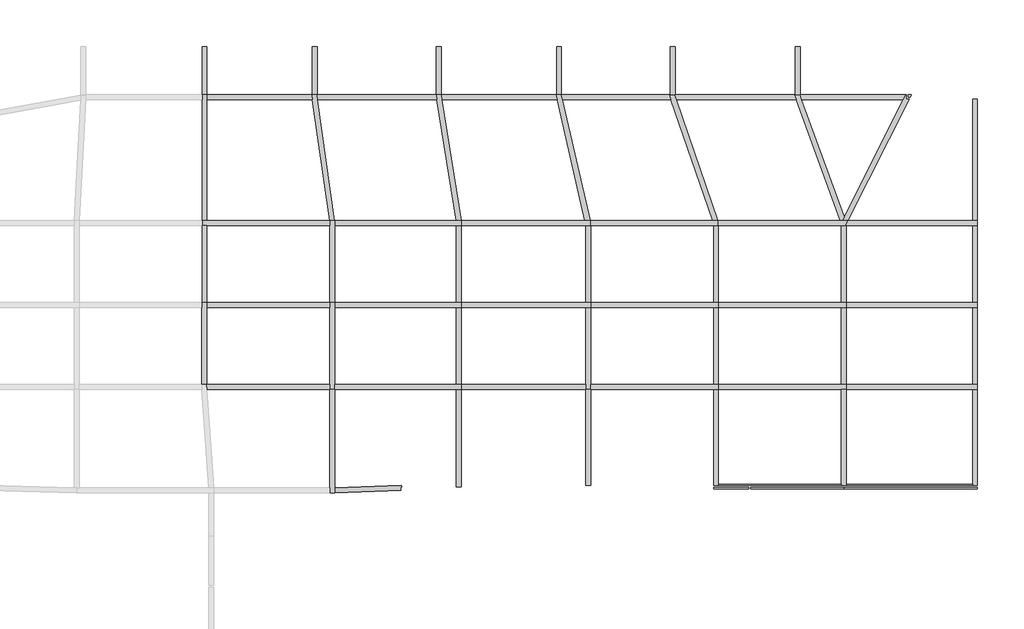
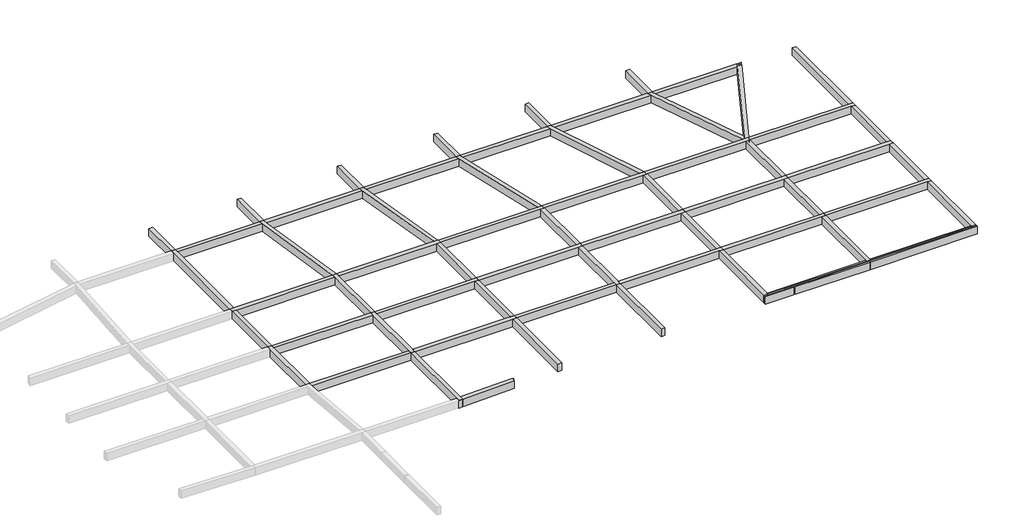
# One storey, part 15 of 15: 61 beams.
"""IFC4 building model written with IfcOpenShell, lengths in millimetres."""

from ifc_helpers import new_model, si_unit, frame, origin, place, context, project, spatial, polyline, outline, extrude, faceted_brep, element, save

model = new_model("IFC4")

# Units and contexts
model_context = context("Model", 3, world=origin())
ifc_project = project(units=[si_unit("LENGTHUNIT", "METRE", prefix="MILLI")], contexts=[model_context])

# Site, building, storey
site = spatial("IfcSite", under=ifc_project)
building = spatial("IfcBuilding", under=site)
storey = spatial("IfcBuildingStorey", under=building, Name="层高", Elevation=3300.0)

# Beams
placement = place(None, origin())
element("IfcBeam", 1, ObjectType="混凝土 - 矩形梁 : KL_beam", at=placement, inside=storey, context=model_context, shape_type="Brep", body=[
    faceted_brep([(266349.8041274, 106691.6486698, 3300.0), (266649.8041274, 106691.6486698, 3300.0), (266649.8041274, 106991.6486698, 3300.0), (266649.8041274, 111691.6486698, 3300.0), (266649.8041274, 111991.6486698, 3300.0), (266349.8041274, 111991.6486698, 3300.0), (266349.8041274, 111691.6486698, 3300.0), (266349.8041274, 106991.6486698, 3300.0), (266649.8041274, 106691.6486698, 2700.0), (266649.8041274, 106991.6486698, 2700.0), (266649.8041274, 111691.6486698, 2700.0), (266649.8041274, 111991.6486698, 2700.0), (266349.8041274, 106691.6486698, 2700.0), (266349.8041274, 106991.6486698, 2700.0), (266349.8041274, 111691.6486698, 2700.0), (266349.8041274, 111991.6486698, 2700.0)], [[[0, 1, 2, 3, 4, 5, 6, 7]], [[1, 8, 9, 10, 11, 4, 3, 2]], [[8, 12, 13, 14, 15, 11, 10, 9]], [[12, 0, 7, 6, 5, 15, 14, 13]], [[1, 0, 12, 8]], [[5, 4, 11, 15]]]),
])
element("IfcBeam", 2, ObjectType="混凝土 - 矩形梁 : KL_beam", at=placement, inside=storey, context=model_context, shape_type="Brep", body=[
    faceted_brep([(274370.4678588, 106691.6486698, 3300.0), (274370.4678588, 106991.6486698, 3300.0), (274070.4678588, 106991.6486698, 3300.0), (266649.8041274, 106991.6486698, 3300.0), (266649.8041274, 106691.6486698, 3300.0), (274070.4678588, 106691.6486698, 3300.0), (274370.4678588, 106991.6486698, 2700.0), (274070.4678588, 106991.6486698, 2700.0), (266649.8041274, 106991.6486698, 2700.0), (274370.4678588, 106691.6486698, 2700.0), (274070.4678588, 106691.6486698, 2700.0), (266649.8041274, 106691.6486698, 2700.0)], [[[0, 1, 2, 3, 4, 5]], [[1, 6, 7, 8, 3, 2]], [[6, 9, 10, 11, 8, 7]], [[9, 0, 5, 4, 11, 10]], [[4, 3, 8, 11]], [[1, 0, 9, 6]]]),
])
element("IfcBeam", 3, ObjectType="混凝土 - 矩形梁 : KL_beam", at=placement, inside=storey, context=model_context, shape_type="Brep", body=[
    faceted_brep([(274370.4678588, 111691.6486698, 3300.0), (274370.4678588, 111991.6486698, 3300.0), (274070.4678588, 111991.6486698, 3300.0), (266649.8041274, 111991.6486698, 3300.0), (266649.8041274, 111691.6486698, 3300.0), (274070.4678588, 111691.6486698, 3300.0), (274370.4678588, 111691.6486698, 2700.0), (266649.8041274, 111691.6486698, 2700.0), (274070.4678588, 111691.6486698, 2700.0), (274370.4678588, 111991.6486698, 2700.0), (266649.8041274, 111991.6486698, 2700.0), (274070.4678588, 111991.6486698, 2700.0)], [[[0, 1, 2, 3, 4, 5]], [[6, 0, 5, 4, 7, 8]], [[9, 6, 8, 7, 10, 11]], [[1, 9, 11, 10, 3, 2]], [[4, 3, 10, 7]], [[1, 0, 6, 9]]]),
])
element("IfcBeam", 4, ObjectType="混凝土 - 矩形梁 : KL_beam", at=placement, inside=storey, context=model_context, shape_type="SweptSolid", body=[
    extrude(outline(polyline([(274370.4678588, 106991.6486698), (274070.4678588, 106991.6486698), (274070.4678588, 111691.6486698), (274370.4678588, 111691.6486698), (274370.4678588, 106991.6486698)])), frame((0.0, 0.0, 2700.0), z_axis=(0.0, 0.0, 1.0), x_axis=(1.0, 0.0, 0.0)), (0.0, 0.0, 1.0), 600.0),
])
element("IfcBeam", 5, ObjectType="混凝土 - 矩形梁 : KL_beam", at=placement, inside=storey, context=model_context, shape_type="Brep", body=[
    faceted_brep([(266349.8041274, 100396.7953536, 3300.0), (266649.8041274, 100396.7953536, 3300.0), (266649.8041274, 100696.9782169, 3300.0), (266649.8041274, 106691.6486698, 3300.0), (266349.8041274, 106691.6486698, 3300.0), (266349.8041274, 100691.6486698, 3300.0), (266349.8041274, 100396.7953536, 2700.0), (266349.8041274, 106691.6486698, 2700.0), (266349.8041274, 100691.6486698, 2700.0), (266649.8041274, 100396.7953536, 2700.0), (266649.8041274, 106691.6486698, 2700.0), (266649.8041274, 100696.9782169, 2700.0)], [[[0, 1, 2, 3, 4, 5]], [[6, 0, 5, 4, 7, 8]], [[9, 6, 8, 7, 10, 11]], [[1, 9, 11, 10, 3, 2]], [[4, 3, 10, 7]], [[1, 0, 6, 9]]]),
])
element("IfcBeam", 6, ObjectType="混凝土 - 矩形梁 : KL_beam", at=placement, inside=storey, context=model_context, shape_type="Brep", body=[
    faceted_brep([(270716.2250579, 100838.9807649, 2700.0), (270716.2250579, 100838.9807649, 3300.0), (270719.5879307, 100742.6806889, 3300.0), (270719.5879307, 100742.6806889, 2700.0), (266649.8041274, 100696.9782169, 3300.0), (266649.8041274, 100396.7953536, 3300.0), (270661.6831769, 100536.8932571, 3300.0), (270661.6831769, 100742.6806889, 3300.0), (266349.8041274, 100386.3191227, 3300.0), (266349.8041274, 100386.3191227, 2700.0), (266649.8041274, 100396.7953536, 2700.0), (270661.6831769, 100536.8932571, 2700.0), (266649.8041274, 100696.9782169, 2700.0), (270661.6831769, 100742.6806889, 2700.0), (266349.8041274, 100391.6486698, 3300.0), (266349.8041274, 100396.7953536, 3300.0), (266349.8041274, 100396.7953536, 2700.0), (266349.8041274, 100391.6486698, 2700.0)], [[[0, 1, 2, 3]], [[1, 4, 5, 6, 7, 2]], [[8, 9, 10, 11, 6, 5]], [[12, 0, 3, 13, 11, 10]], [[1, 0, 12, 4]], [[9, 8, 14, 15, 16, 17]], [[10, 5, 4, 12]], [[5, 10, 16, 15]], [[15, 14, 8, 5]], [[10, 9, 17, 16]], [[13, 7, 6, 11]], [[7, 13, 3, 2]]]),
])
element("IfcBeam", 7, ObjectType="混凝土 - 矩形梁 : KL_beam", at=placement, inside=storey, context=model_context, shape_type="SweptSolid", body=[
    extrude(outline(polyline([(274070.4678588, 106691.6486698), (274370.4678588, 106691.6486698), (274370.4678588, 100742.6806889), (274070.4678588, 100742.6806889), (274070.4678588, 106691.6486698)])), frame((0.0, 0.0, 2700.0), z_axis=(0.0, 0.0, 1.0), x_axis=(1.0, 0.0, 0.0)), (0.0, 0.0, 1.0), 600.0),
])
element("IfcBeam", 8, ObjectType="混凝土 - 矩形梁 : KL_beam", at=placement, inside=storey, context=model_context, shape_type="Brep", body=[
    faceted_brep([(266349.8041274, 106691.6486698, 3300.0), (266349.8041274, 106991.6486698, 3300.0), (258831.1501343, 106991.6486698, 3300.0), (258821.0273972, 106991.6486698, 3300.0), (258842.0054408, 106691.6486698, 3300.0), (266349.8041274, 106991.6486698, 2700.0), (258831.1501343, 106991.6486698, 2700.0), (258821.0273972, 106991.6486698, 2700.0), (266349.8041274, 106691.6486698, 2700.0), (258842.0054408, 106691.6486698, 2700.0)], [[[0, 1, 2, 3, 4]], [[1, 5, 6, 7, 3, 2]], [[5, 8, 9, 7, 6]], [[8, 0, 4, 9]], [[1, 0, 8, 5]], [[4, 3, 7, 9]]]),
])
element("IfcBeam", 9, ObjectType="混凝土 - 矩形梁 : KL_beam", at=placement, inside=storey, context=model_context, shape_type="Brep", body=[
    faceted_brep([(258831.1501343, 106991.6486698, 3300.0), (258831.1501343, 106991.6486698, 2700.0), (258831.1501343, 111691.6486698, 2700.0), (258831.1501343, 111991.6486698, 2700.0), (258831.1501343, 111991.6486698, 3300.0), (258831.1501343, 111691.6486698, 3300.0), (258549.8041274, 111991.6486698, 3300.0), (258531.1501343, 111991.6486698, 3300.0), (258531.1501343, 111691.6486698, 3300.0), (258531.1501343, 106991.6486698, 3300.0), (258821.0273972, 106991.6486698, 3300.0), (258531.1501343, 111991.6486698, 2700.0), (258549.8041274, 111991.6486698, 2700.0), (258821.0273972, 106991.6486698, 2700.0), (258531.1501343, 106991.6486698, 2700.0), (258531.1501343, 111691.6486698, 2700.0)], [[[0, 1, 2, 3, 4, 5]], [[4, 6, 7, 8, 9, 10, 0, 5]], [[11, 12, 3, 2, 1, 13, 14, 15]], [[7, 11, 15, 14, 9, 8]], [[1, 0, 10, 9, 14, 13]], [[7, 6, 4, 3, 12, 11]]]),
])
element("IfcBeam", 10, ObjectType="混凝土 - 矩形梁 : KL_beam", at=placement, inside=storey, context=model_context, shape_type="Brep", body=[
    faceted_brep([(266349.8041274, 111691.6486698, 3300.0), (266349.8041274, 111991.6486698, 3300.0), (258849.8041274, 111991.6486698, 3300.0), (258831.1501343, 111991.6486698, 3300.0), (258831.1501343, 111691.6486698, 3300.0), (266349.8041274, 111691.6486698, 2700.0), (258831.1501343, 111691.6486698, 2700.0), (266349.8041274, 111991.6486698, 2700.0), (258831.1501343, 111991.6486698, 2700.0), (258849.8041274, 111991.6486698, 2700.0)], [[[0, 1, 2, 3, 4]], [[5, 0, 4, 6]], [[7, 5, 6, 8, 9]], [[1, 7, 9, 8, 3, 2]], [[1, 0, 5, 7]], [[4, 3, 8, 6]]]),
])
element("IfcBeam", 11, ObjectType="混凝土 - 矩形梁 : KL_beam", at=placement, inside=storey, context=model_context, shape_type="Brep", body=[
    faceted_brep([(266649.8041274, 116991.6486698, 3300.0), (266630.197138, 116991.6486698, 3300.0), (266349.8041274, 116991.6486698, 3300.0), (266349.8041274, 116691.6486698, 3300.0), (266349.8041274, 111991.6486698, 3300.0), (266649.8041274, 111991.6486698, 3300.0), (266649.8041274, 116691.6486698, 3300.0), (266649.8041274, 116852.1376916, 3300.0), (266649.8041274, 116991.6486698, 2700.0), (266649.8041274, 111991.6486698, 2700.0), (266649.8041274, 116691.6486698, 2700.0), (266649.8041274, 116852.1376916, 2700.0), (266349.8041274, 116991.6486698, 2700.0), (266630.197138, 116991.6486698, 2700.0), (266349.8041274, 111991.6486698, 2700.0), (266349.8041274, 116691.6486698, 2700.0)], [[[0, 1, 2, 3, 4, 5, 6, 7]], [[8, 0, 7, 6, 5, 9, 10, 11]], [[12, 13, 8, 11, 10, 9, 14, 15]], [[2, 12, 15, 14, 4, 3]], [[5, 4, 14, 9]], [[2, 1, 0, 8, 13, 12]]]),
])
element("IfcBeam", 12, ObjectType="混凝土 - 矩形梁 : KL_beam", at=placement, inside=storey, context=model_context, shape_type="Brep", body=[
    faceted_brep([(258549.8041274, 116991.6486698, 3300.0), (258549.8041274, 116691.6486698, 3300.0), (258849.8041274, 116691.6486698, 3300.0), (266349.8041274, 116691.6486698, 3300.0), (266349.8041274, 116991.6486698, 3300.0), (266327.2488663, 116991.6486698, 3300.0), (258849.8041274, 116991.6486698, 3300.0), (258549.8041274, 116991.6486698, 2700.0), (266349.8041274, 116991.6486698, 2700.0), (266327.2488663, 116991.6486698, 2700.0), (258849.8041274, 116991.6486698, 2700.0), (258549.8041274, 116691.6486698, 2700.0), (266349.8041274, 116691.6486698, 2700.0), (258849.8041274, 116691.6486698, 2700.0)], [[[0, 1, 2, 3, 4, 5, 6]], [[7, 0, 6, 5, 4, 8, 9, 10]], [[11, 7, 10, 9, 8, 12, 13]], [[1, 11, 13, 12, 3, 2]], [[4, 3, 12, 8]], [[1, 0, 7, 11]]]),
])
element("IfcBeam", 13, ObjectType="混凝土 - 矩形梁 : KL_beam", at=placement, inside=storey, context=model_context, shape_type="Brep", body=[
    faceted_brep([(258549.8041274, 111991.6486698, 3300.0), (258831.1501343, 111991.6486698, 3300.0), (258849.8041274, 111991.6486698, 3300.0), (258849.8041274, 116691.6486698, 3300.0), (258549.8041274, 116691.6486698, 3300.0), (258549.8041274, 111991.6486698, 2700.0), (258549.8041274, 116691.6486698, 2700.0), (258849.8041274, 111991.6486698, 2700.0), (258831.1501343, 111991.6486698, 2700.0), (258849.8041274, 116691.6486698, 2700.0)], [[[0, 1, 2, 3, 4]], [[5, 0, 4, 6]], [[7, 8, 5, 6, 9]], [[2, 7, 9, 3]], [[0, 5, 8, 7, 2, 1]], [[4, 3, 9, 6]]]),
])
element("IfcBeam", 14, ObjectType="混凝土 - 矩形梁 : KL_beam", at=placement, inside=storey, context=model_context, shape_type="Brep", body=[
    faceted_brep([(258849.8041274, 124681.0960874, 3300.0), (258549.8041274, 124681.0960874, 3300.0), (258549.8041274, 124381.0960874, 3300.0), (258549.8041274, 116991.6486698, 3300.0), (258849.8041274, 116991.6486698, 3300.0), (258849.8041274, 124381.0960874, 3300.0), (258849.8041274, 124681.0960874, 2700.0), (258849.8041274, 116991.6486698, 2700.0), (258849.8041274, 124381.0960874, 2700.0), (258549.8041274, 124681.0960874, 2700.0), (258549.8041274, 116991.6486698, 2700.0), (258549.8041274, 124381.0960874, 2700.0)], [[[0, 1, 2, 3, 4, 5]], [[6, 0, 5, 4, 7, 8]], [[9, 6, 8, 7, 10, 11]], [[1, 9, 11, 10, 3, 2]], [[4, 3, 10, 7]], [[1, 0, 6, 9]]]),
])
element("IfcBeam", 15, ObjectType="混凝土 - 矩形梁 : KL_beam", at=placement, inside=storey, context=model_context, shape_type="Brep", body=[
    faceted_brep([(266327.2488663, 116991.6486698, 3300.0), (266349.8041274, 116991.6486698, 3300.0), (266630.197138, 116991.6486698, 3300.0), (265591.67803, 124381.0960874, 3300.0), (265549.5157796, 124681.0960874, 3300.0), (265269.1227689, 124681.0960874, 3300.0), (265246.5675078, 124681.0960874, 3300.0), (265288.7297582, 124381.0960874, 3300.0), (266630.197138, 116991.6486698, 2700.0), (265591.67803, 124381.0960874, 2700.0), (265549.5157796, 124681.0960874, 2700.0), (266349.8041274, 116991.6486698, 2700.0), (266327.2488663, 116991.6486698, 2700.0), (265288.7297582, 124381.0960874, 2700.0), (265246.5675078, 124681.0960874, 2700.0), (265269.1227689, 124681.0960874, 2700.0)], [[[0, 1, 2, 3, 4, 5, 6, 7]], [[2, 8, 9, 10, 4, 3]], [[8, 11, 12, 13, 14, 15, 10, 9]], [[6, 14, 13, 12, 0, 7]], [[0, 12, 11, 8, 2, 1]], [[6, 5, 4, 10, 15, 14]]]),
    faceted_brep([(266672.3593884, 116691.6486698, 2700.0), (266672.3593884, 116691.6486698, 3300.0), (266649.8041274, 116691.6486698, 3300.0), (266649.8041274, 116691.6486698, 2700.0), (266649.8041274, 116852.1376916, 3300.0), (266649.8041274, 116852.1376916, 2700.0)], [[[0, 1, 2, 3]], [[2, 4, 5, 3]], [[4, 2, 1]], [[1, 0, 5, 4]], [[3, 5, 0]]]),
])
element("IfcBeam", 16, ObjectType="混凝土 - 矩形梁 : KL_beam", at=placement, inside=storey, context=model_context, shape_type="Brep", body=[
    faceted_brep([(274370.4678588, 116691.6486698, 3300.0), (274370.4678588, 116991.6486698, 3300.0), (274348.5799616, 116991.6486698, 3300.0), (274044.8404239, 116991.6486698, 3300.0), (266649.8041274, 116991.6486698, 3300.0), (266649.8041274, 116852.1376916, 3300.0), (266672.3593884, 116691.6486698, 3300.0), (274070.4678588, 116691.6486698, 3300.0), (274370.4678588, 116691.6486698, 2700.0), (266672.3593884, 116691.6486698, 2700.0), (274070.4678588, 116691.6486698, 2700.0), (274370.4678588, 116991.6486698, 2700.0), (266649.8041274, 116852.1376916, 2700.0), (266649.8041274, 116991.6486698, 2700.0), (274044.8404239, 116991.6486698, 2700.0), (274348.5799616, 116991.6486698, 2700.0)], [[[0, 1, 2, 3, 4, 5, 6, 7]], [[8, 0, 7, 6, 9, 10]], [[11, 8, 10, 9, 12, 13, 14, 15]], [[13, 4, 3, 2, 1, 11, 15, 14]], [[4, 13, 12, 5]], [[6, 5, 12, 9]], [[1, 0, 8, 11]]]),
])
element("IfcBeam", 17, ObjectType="混凝土 - 矩形梁 : KL_beam", at=placement, inside=storey, context=model_context, shape_type="SweptSolid", body=[
    extrude(outline(polyline([(274370.4678588, 111991.6486698), (274070.4678588, 111991.6486698), (274070.4678588, 116691.6486698), (274370.4678588, 116691.6486698), (274370.4678588, 111991.6486698)])), frame((0.0, 0.0, 2700.0), z_axis=(0.0, 0.0, 1.0), x_axis=(1.0, 0.0, 0.0)), (0.0, 0.0, 1.0), 600.0),
])
element("IfcBeam", 18, ObjectType="混凝土 - 矩形梁 : KL_beam", at=placement, inside=storey, context=model_context, shape_type="Brep", body=[
    faceted_brep([(282219.0254303, 116691.6486698, 3300.0), (282219.0254303, 116991.6486698, 3300.0), (281911.134198, 116991.6486698, 3300.0), (274370.4678588, 116991.6486698, 3300.0), (274370.4678588, 116691.6486698, 3300.0), (281949.7100428, 116691.6486698, 3300.0), (282219.0254303, 116691.6486698, 2700.0), (274370.4678588, 116691.6486698, 2700.0), (281949.7100428, 116691.6486698, 2700.0), (282219.0254303, 116991.6486698, 2700.0), (274370.4678588, 116991.6486698, 2700.0), (281911.134198, 116991.6486698, 2700.0)], [[[0, 1, 2, 3, 4, 5]], [[6, 0, 5, 4, 7, 8]], [[9, 6, 8, 7, 10, 11]], [[1, 9, 11, 10, 3, 2]], [[4, 3, 10, 7]], [[1, 0, 6, 9]]]),
])
element("IfcBeam", 19, ObjectType="混凝土 - 矩形梁 : KL_beam", at=placement, inside=storey, context=model_context, shape_type="Brep", body=[
    faceted_brep([(290006.8166962, 116691.6486698, 3300.0), (290006.8166962, 116991.6486698, 3300.0), (289689.5304919, 116991.6486698, 3300.0), (282219.0254303, 116991.6486698, 3300.0), (282219.0254303, 116691.6486698, 3300.0), (282249.7100428, 116691.6486698, 3300.0), (289749.8227361, 116691.6486698, 3300.0), (290006.8166962, 116691.6486698, 2700.0), (282219.0254303, 116691.6486698, 2700.0), (282249.7100428, 116691.6486698, 2700.0), (289749.8227361, 116691.6486698, 2700.0), (290006.8166962, 116991.6486698, 2700.0), (282219.0254303, 116991.6486698, 2700.0), (289689.5304919, 116991.6486698, 2700.0)], [[[0, 1, 2, 3, 4, 5, 6]], [[7, 0, 6, 5, 4, 8, 9, 10]], [[11, 7, 10, 9, 8, 12, 13]], [[1, 11, 13, 12, 3, 2]], [[4, 3, 12, 8]], [[1, 0, 7, 11]]]),
])
element("IfcBeam", 20, ObjectType="混凝土 - 矩形梁 : KL_beam", at=placement, inside=storey, context=model_context, shape_type="Brep", body=[
    faceted_brep([(297792.1399936, 116691.6486698, 3300.0), (297943.4797534, 116991.6486698, 3300.0), (297607.4682611, 116991.6486698, 3300.0), (297485.5819263, 116991.6486698, 3300.0), (290006.8166962, 116991.6486698, 3300.0), (290006.8166962, 116691.6486698, 3300.0), (290049.8227361, 116691.6486698, 3300.0), (297549.8041274, 116691.6486698, 3300.0), (297792.1399936, 116691.6486698, 2700.0), (290006.8166962, 116691.6486698, 2700.0), (290049.8227361, 116691.6486698, 2700.0), (297549.8041274, 116691.6486698, 2700.0), (297943.4797534, 116991.6486698, 2700.0), (290006.8166962, 116991.6486698, 2700.0), (297485.5819263, 116991.6486698, 2700.0), (297607.4682611, 116991.6486698, 2700.0)], [[[0, 1, 2, 3, 4, 5, 6, 7]], [[8, 0, 7, 6, 5, 9, 10, 11]], [[12, 8, 11, 10, 9, 13, 14, 15]], [[1, 12, 15, 14, 13, 4, 3, 2]], [[5, 4, 13, 9]], [[1, 0, 8, 12]]]),
])
element("IfcBeam", 21, ObjectType="混凝土 - 矩形梁 : KL_beam", at=placement, inside=storey, context=model_context, shape_type="Brep", body=[
    faceted_brep([(297943.4797534, 116991.6486698, 3300.0), (297792.1399936, 116691.6486698, 3300.0), (297849.8041274, 116691.6486698, 3300.0), (305549.8041274, 116691.6486698, 3300.0), (305849.8041274, 116691.6486698, 3300.0), (305849.8041274, 116991.6486698, 3300.0), (305549.8041274, 116991.6486698, 3300.0), (297792.1399936, 116691.6486698, 2700.0), (297849.8041274, 116691.6486698, 2700.0), (305549.8041274, 116691.6486698, 2700.0), (305849.8041274, 116691.6486698, 2700.0), (297943.4797534, 116991.6486698, 2700.0), (305549.8041274, 116991.6486698, 2700.0), (305849.8041274, 116991.6486698, 2700.0)], [[[0, 1, 2, 3, 4, 5, 6]], [[1, 7, 8, 9, 10, 4, 3, 2]], [[7, 11, 12, 13, 10, 9, 8]], [[11, 0, 6, 5, 13, 12]], [[1, 0, 11, 7]], [[5, 4, 10, 13]]]),
])
element("IfcBeam", 22, ObjectType="混凝土 - 矩形梁 : KL_beam", at=placement, inside=storey, context=model_context, shape_type="Brep", body=[
    faceted_brep([(301822.5435038, 124681.0960874, 3300.0), (301617.9590704, 124681.0960874, 3300.0), (301617.9590704, 124549.6486698, 3300.0), (301756.2327685, 124549.6486698, 3300.0), (301822.5435038, 124681.0960874, 2700.0), (301756.2327685, 124549.6486698, 2700.0), (301617.9590704, 124681.0960874, 2700.0), (301617.9590704, 124549.6486698, 2700.0)], [[[0, 1, 2, 3]], [[4, 0, 3, 5]], [[6, 4, 5, 7]], [[1, 6, 7, 2]], [[3, 2, 7, 5]], [[0, 4, 6, 1]]]),
    faceted_brep([(297607.4682611, 116991.6486698, 2700.0), (297607.4682611, 116991.6486698, 3300.0), (297722.1167805, 117218.9158192, 3300.0), (301335.1922518, 124381.0960874, 3300.0), (301486.5320116, 124681.0960874, 3300.0), (301486.5320116, 124681.0960874, 2700.0), (301335.1922518, 124381.0960874, 2700.0), (297722.1167805, 117218.9158192, 2700.0), (297943.4797534, 116991.6486698, 3300.0), (297943.4797534, 116991.6486698, 2700.0), (301497.9590704, 124681.0960874, 3300.0), (301497.9590704, 124681.0960874, 2700.0), (301497.9590704, 124429.6486698, 3300.0), (301497.9590704, 124429.6486698, 2700.0), (301695.6968645, 124429.6486698, 3300.0), (301695.6968645, 124429.6486698, 2700.0)], [[[0, 1, 2, 3, 4, 5, 6, 7]], [[8, 1, 0, 9]], [[5, 4, 10, 11]], [[12, 13, 11, 10]], [[13, 12, 14, 15]], [[1, 8, 14, 12, 10, 4, 3, 2]], [[8, 9, 15, 14]], [[9, 0, 7, 6, 5, 11, 13, 15]]]),
])
element("IfcBeam", 23, ObjectType="混凝土 - 矩形梁 : KL_beam", at=placement, inside=storey, context=model_context, shape_type="Brep", body=[
    faceted_brep([(297485.5819263, 116991.6486698, 3300.0), (297607.4682611, 116991.6486698, 3300.0), (297722.1167805, 117218.9158192, 3300.0), (295115.2963504, 124381.0960874, 3300.0), (295006.1052801, 124681.0960874, 3300.0), (294751.0741494, 124681.0960874, 3300.0), (294686.8519484, 124681.0960874, 3300.0), (294796.0430187, 124381.0960874, 3300.0), (297722.1167805, 117218.9158192, 2700.0), (295115.2963504, 124381.0960874, 2700.0), (295006.1052801, 124681.0960874, 2700.0), (297607.4682611, 116991.6486698, 2700.0), (297485.5819263, 116991.6486698, 2700.0), (294796.0430187, 124381.0960874, 2700.0), (294686.8519484, 124681.0960874, 2700.0), (294751.0741494, 124681.0960874, 2700.0)], [[[0, 1, 2, 3, 4, 5, 6, 7]], [[2, 8, 9, 10, 4, 3]], [[11, 12, 13, 14, 15, 10, 9, 8]], [[12, 0, 7, 6, 14, 13]], [[0, 12, 11, 1]], [[2, 1, 11, 8]], [[6, 5, 4, 10, 15, 14]]]),
])
element("IfcBeam", 24, ObjectType="混凝土 - 矩形梁 : KL_beam", at=placement, inside=storey, context=model_context, shape_type="Brep", body=[
    faceted_brep([(287359.1276194, 124681.0960874, 3300.0), (287102.1336592, 124681.0960874, 3300.0), (287041.8414151, 124681.0960874, 3300.0), (287145.139699, 124381.0960874, 3300.0), (289689.5304919, 116991.6486698, 3300.0), (290006.8166962, 116991.6486698, 3300.0), (287462.4259034, 124381.0960874, 3300.0), (287359.1276194, 124681.0960874, 2700.0), (290006.8166962, 116991.6486698, 2700.0), (287462.4259034, 124381.0960874, 2700.0), (287041.8414151, 124681.0960874, 2700.0), (287102.1336592, 124681.0960874, 2700.0), (289689.5304919, 116991.6486698, 2700.0), (287145.139699, 124381.0960874, 2700.0)], [[[0, 1, 2, 3, 4, 5, 6]], [[7, 0, 6, 5, 8, 9]], [[10, 11, 7, 9, 8, 12, 13]], [[2, 10, 13, 12, 4, 3]], [[5, 4, 12, 8]], [[2, 1, 0, 7, 11, 10]]]),
])
element("IfcBeam", 25, ObjectType="混凝土 - 矩形梁 : KL_beam", at=placement, inside=storey, context=model_context, shape_type="Brep", body=[
    faceted_brep([(280443.7766143, 124681.0960874, 3300.0), (280174.4612268, 124681.0960874, 3300.0), (280135.8853819, 124681.0960874, 3300.0), (280205.1458393, 124381.0960874, 3300.0), (281911.134198, 116991.6486698, 3300.0), (282219.0254303, 116991.6486698, 3300.0), (280513.0370716, 124381.0960874, 3300.0), (280443.7766143, 124681.0960874, 2700.0), (282219.0254303, 116991.6486698, 2700.0), (280513.0370716, 124381.0960874, 2700.0), (280135.8853819, 124681.0960874, 2700.0), (280174.4612268, 124681.0960874, 2700.0), (281911.134198, 116991.6486698, 2700.0), (280205.1458393, 124381.0960874, 2700.0)], [[[0, 1, 2, 3, 4, 5, 6]], [[7, 0, 6, 5, 8, 9]], [[10, 11, 7, 9, 8, 12, 13]], [[2, 10, 13, 12, 4, 3]], [[5, 4, 12, 8]], [[2, 1, 0, 7, 11, 10]]]),
])
element("IfcBeam", 26, ObjectType="混凝土 - 矩形梁 : KL_beam", at=placement, inside=storey, context=model_context, shape_type="Brep", body=[
    faceted_brep([(274044.8404239, 116991.6486698, 3300.0), (274070.4678588, 116991.6486698, 3300.0), (274348.5799616, 116991.6486698, 3300.0), (273178.2064681, 124381.0960874, 3300.0), (273130.691136, 124681.0960874, 3300.0), (272852.5790331, 124681.0960874, 3300.0), (272826.9515982, 124681.0960874, 3300.0), (272874.4669303, 124381.0960874, 3300.0), (274348.5799616, 116991.6486698, 2700.0), (273178.2064681, 124381.0960874, 2700.0), (273130.691136, 124681.0960874, 2700.0), (274070.4678588, 116991.6486698, 2700.0), (274044.8404239, 116991.6486698, 2700.0), (272874.4669303, 124381.0960874, 2700.0), (272826.9515982, 124681.0960874, 2700.0), (272852.5790331, 124681.0960874, 2700.0)], [[[0, 1, 2, 3, 4, 5, 6, 7]], [[2, 8, 9, 10, 4, 3]], [[8, 11, 12, 13, 14, 15, 10, 9]], [[12, 0, 7, 6, 14, 13]], [[8, 2, 1, 0, 12, 11]], [[6, 5, 4, 10, 15, 14]]]),
])
element("IfcBeam", 27, ObjectType="混凝土 - 矩形梁 : KL_beam", at=placement, inside=storey, context=model_context, shape_type="Brep", body=[
    faceted_brep([(282249.7100428, 111691.6486698, 3300.0), (282249.7100428, 111991.6486698, 3300.0), (281949.7100428, 111991.6486698, 3300.0), (274370.4678588, 111991.6486698, 3300.0), (274370.4678588, 111691.6486698, 3300.0), (281949.7100428, 111691.6486698, 3300.0), (282249.7100428, 111691.6486698, 2700.0), (274370.4678588, 111691.6486698, 2700.0), (281949.7100428, 111691.6486698, 2700.0), (282249.7100428, 111991.6486698, 2700.0), (274370.4678588, 111991.6486698, 2700.0), (281949.7100428, 111991.6486698, 2700.0)], [[[0, 1, 2, 3, 4, 5]], [[6, 0, 5, 4, 7, 8]], [[9, 6, 8, 7, 10, 11]], [[1, 9, 11, 10, 3, 2]], [[4, 3, 10, 7]], [[1, 0, 6, 9]]]),
])
element("IfcBeam", 28, ObjectType="混凝土 - 矩形梁 : KL_beam", at=placement, inside=storey, context=model_context, shape_type="Brep", body=[
    faceted_brep([(290049.8227361, 111691.6486698, 3300.0), (290049.8227361, 111991.6486698, 3300.0), (289749.8227361, 111991.6486698, 3300.0), (282249.7100428, 111991.6486698, 3300.0), (282249.7100428, 111691.6486698, 3300.0), (289749.8227361, 111691.6486698, 3300.0), (290049.8227361, 111691.6486698, 2700.0), (282249.7100428, 111691.6486698, 2700.0), (289749.8227361, 111691.6486698, 2700.0), (290049.8227361, 111991.6486698, 2700.0), (282249.7100428, 111991.6486698, 2700.0), (289749.8227361, 111991.6486698, 2700.0)], [[[0, 1, 2, 3, 4, 5]], [[6, 0, 5, 4, 7, 8]], [[9, 6, 8, 7, 10, 11]], [[1, 9, 11, 10, 3, 2]], [[1, 0, 6, 9]], [[4, 3, 10, 7]]]),
])
element("IfcBeam", 29, ObjectType="混凝土 - 矩形梁 : KL_beam", at=placement, inside=storey, context=model_context, shape_type="Brep", body=[
    faceted_brep([(297849.8041274, 111691.6486698, 3300.0), (297849.8041274, 111991.6486698, 3300.0), (297549.8041274, 111991.6486698, 3300.0), (290049.8227361, 111991.6486698, 3300.0), (290049.8227361, 111691.6486698, 3300.0), (297549.8041274, 111691.6486698, 3300.0), (297849.8041274, 111691.6486698, 2700.0), (290049.8227361, 111691.6486698, 2700.0), (297549.8041274, 111691.6486698, 2700.0), (297849.8041274, 111991.6486698, 2700.0), (290049.8227361, 111991.6486698, 2700.0), (297549.8041274, 111991.6486698, 2700.0)], [[[0, 1, 2, 3, 4, 5]], [[6, 0, 5, 4, 7, 8]], [[9, 6, 8, 7, 10, 11]], [[1, 9, 11, 10, 3, 2]], [[4, 3, 10, 7]], [[1, 0, 6, 9]]]),
])
element("IfcBeam", 30, ObjectType="混凝土 - 矩形梁 : KL_beam", at=placement, inside=storey, context=model_context, shape_type="Brep", body=[
    faceted_brep([(290049.8227361, 116691.6486698, 3300.0), (290006.8166962, 116691.6486698, 3300.0), (289749.8227361, 116691.6486698, 3300.0), (289749.8227361, 111991.6486698, 3300.0), (290049.8227361, 111991.6486698, 3300.0), (290049.8227361, 116691.6486698, 2700.0), (290049.8227361, 111991.6486698, 2700.0), (289749.8227361, 116691.6486698, 2700.0), (290006.8166962, 116691.6486698, 2700.0), (289749.8227361, 111991.6486698, 2700.0)], [[[0, 1, 2, 3, 4]], [[5, 0, 4, 6]], [[7, 8, 5, 6, 9]], [[2, 7, 9, 3]], [[7, 2, 1, 0, 5, 8]], [[4, 3, 9, 6]]]),
])
element("IfcBeam", 31, ObjectType="混凝土 - 矩形梁 : KL_beam", at=placement, inside=storey, context=model_context, shape_type="Brep", body=[
    faceted_brep([(282249.7100428, 116691.6486698, 3300.0), (282219.0254303, 116691.6486698, 3300.0), (281949.7100428, 116691.6486698, 3300.0), (281949.7100428, 111991.6486698, 3300.0), (282249.7100428, 111991.6486698, 3300.0), (282249.7100428, 116691.6486698, 2700.0), (282249.7100428, 111991.6486698, 2700.0), (281949.7100428, 116691.6486698, 2700.0), (282219.0254303, 116691.6486698, 2700.0), (281949.7100428, 111991.6486698, 2700.0)], [[[0, 1, 2, 3, 4]], [[5, 0, 4, 6]], [[7, 8, 5, 6, 9]], [[2, 7, 9, 3]], [[7, 2, 1, 0, 5, 8]], [[4, 3, 9, 6]]]),
])
element("IfcBeam", 32, ObjectType="混凝土 - 矩形梁 : KL_beam", at=placement, inside=storey, context=model_context, shape_type="Brep", body=[
    faceted_brep([(281949.7100428, 106691.6486698, 3300.0), (282249.7100428, 106691.6486698, 3300.0), (282249.7100428, 106991.6486698, 3300.0), (282249.7100428, 111691.6486698, 3300.0), (281949.7100428, 111691.6486698, 3300.0), (281949.7100428, 106991.6486698, 3300.0), (282249.7100428, 106691.6486698, 2700.0), (282249.7100428, 106991.6486698, 2700.0), (282249.7100428, 111691.6486698, 2700.0), (281949.7100428, 106691.6486698, 2700.0), (281949.7100428, 106991.6486698, 2700.0), (281949.7100428, 111691.6486698, 2700.0)], [[[0, 1, 2, 3, 4, 5]], [[1, 6, 7, 8, 3, 2]], [[6, 9, 10, 11, 8, 7]], [[9, 0, 5, 4, 11, 10]], [[4, 3, 8, 11]], [[1, 0, 9, 6]]]),
])
element("IfcBeam", 33, ObjectType="混凝土 - 矩形梁 : KL_beam", at=placement, inside=storey, context=model_context, shape_type="SweptSolid", body=[
    extrude(outline(polyline([(281949.7100428, 106691.6486698), (282249.7100428, 106691.6486698), (282249.7100428, 100824.5205023), (281949.7100428, 100824.5205023), (281949.7100428, 106691.6486698)])), frame((0.0, 0.0, 2700.0), z_axis=(0.0, 0.0, 1.0), x_axis=(1.0, 0.0, 0.0)), (0.0, 0.0, 1.0), 600.0),
])
element("IfcBeam", 34, ObjectType="混凝土 - 矩形梁 : KL_beam", at=placement, inside=storey, context=model_context, shape_type="SweptSolid", body=[
    extrude(outline(polyline([(274370.4678588, 106691.6486698), (274370.4678588, 106991.6486698), (281949.7100428, 106991.6486698), (281949.7100428, 106691.6486698), (274370.4678588, 106691.6486698)])), frame((0.0, 0.0, 2700.0), z_axis=(0.0, 0.0, 1.0), x_axis=(1.0, 0.0, 0.0)), (0.0, 0.0, 1.0), 600.0),
])
element("IfcBeam", 35, ObjectType="混凝土 - 矩形梁 : KL_beam", at=placement, inside=storey, context=model_context, shape_type="Brep", body=[
    faceted_brep([(290049.8227361, 106691.6486698, 3300.0), (290049.8227361, 106991.6486698, 3300.0), (289749.8227361, 106991.6486698, 3300.0), (282249.7100428, 106991.6486698, 3300.0), (282249.7100428, 106691.6486698, 3300.0), (289749.8227361, 106691.6486698, 3300.0), (290049.8227361, 106691.6486698, 2700.0), (282249.7100428, 106691.6486698, 2700.0), (289749.8227361, 106691.6486698, 2700.0), (290049.8227361, 106991.6486698, 2700.0), (282249.7100428, 106991.6486698, 2700.0), (289749.8227361, 106991.6486698, 2700.0)], [[[0, 1, 2, 3, 4, 5]], [[6, 0, 5, 4, 7, 8]], [[9, 6, 8, 7, 10, 11]], [[1, 9, 11, 10, 3, 2]], [[4, 3, 10, 7]], [[1, 0, 6, 9]]]),
])
element("IfcBeam", 36, ObjectType="混凝土 - 矩形梁 : KL_beam", at=placement, inside=storey, context=model_context, shape_type="SweptSolid", body=[
    extrude(outline(polyline([(289749.8227361, 111691.6486698), (290049.8227361, 111691.6486698), (290049.8227361, 106991.6486698), (289749.8227361, 106991.6486698), (289749.8227361, 111691.6486698)])), frame((0.0, 0.0, 2700.0), z_axis=(0.0, 0.0, 1.0), x_axis=(1.0, 0.0, 0.0)), (0.0, 0.0, 1.0), 600.0),
])
element("IfcBeam", 37, ObjectType="混凝土 - 矩形梁 : KL_beam", at=placement, inside=storey, context=model_context, shape_type="Brep", body=[
    faceted_brep([(297849.8041274, 106691.6486698, 3300.0), (297849.8041274, 106991.6486698, 3300.0), (297549.8041274, 106991.6486698, 3300.0), (290049.8227361, 106991.6486698, 3300.0), (290049.8227361, 106691.6486698, 3300.0), (297549.8041274, 106691.6486698, 3300.0), (297849.8041274, 106691.6486698, 2700.0), (290049.8227361, 106691.6486698, 2700.0), (297549.8041274, 106691.6486698, 2700.0), (297849.8041274, 106991.6486698, 2700.0), (290049.8227361, 106991.6486698, 2700.0), (297549.8041274, 106991.6486698, 2700.0)], [[[0, 1, 2, 3, 4, 5]], [[6, 0, 5, 4, 7, 8]], [[9, 6, 8, 7, 10, 11]], [[1, 9, 11, 10, 3, 2]], [[4, 3, 10, 7]], [[1, 0, 6, 9]]]),
])
element("IfcBeam", 38, ObjectType="混凝土 - 矩形梁 : KL_beam", at=placement, inside=storey, context=model_context, shape_type="Brep", body=[
    faceted_brep([(290049.8227361, 106691.6486698, 3300.0), (289749.8227361, 106691.6486698, 3300.0), (289749.8227361, 100824.5205023, 3300.0), (290049.8227361, 100824.5205023, 3300.0), (290049.8227361, 100914.5205023, 3300.0), (289749.8227361, 106691.6486698, 2700.0), (289749.8227361, 100824.5205023, 2700.0), (290049.8227361, 106691.6486698, 2700.0), (290049.8227361, 100914.5205023, 2700.0), (290049.8227361, 100824.5205023, 2700.0)], [[[0, 1, 2, 3, 4]], [[1, 5, 6, 2]], [[5, 7, 8, 9, 6]], [[7, 0, 4, 3, 9, 8]], [[1, 0, 7, 5]], [[3, 2, 6, 9]]]),
])
element("IfcBeam", 39, ObjectType="混凝土 - 矩形梁 : KL_beam", at=placement, inside=storey, context=model_context, shape_type="Brep", body=[
    faceted_brep([(297849.8041274, 106691.6486698, 3300.0), (297549.8041274, 106691.6486698, 3300.0), (297549.8041274, 100914.5205023, 3300.0), (297549.8041274, 100824.5205023, 3300.0), (297849.8041274, 100824.5205023, 3300.0), (297849.8041274, 100914.5205023, 3300.0), (297549.8041274, 106691.6486698, 2700.0), (297549.8041274, 100914.5205023, 2700.0), (297549.8041274, 100824.5205023, 2700.0), (297849.8041274, 106691.6486698, 2700.0), (297849.8041274, 100914.5205023, 2700.0), (297849.8041274, 100824.5205023, 2700.0)], [[[0, 1, 2, 3, 4, 5]], [[1, 6, 7, 8, 3, 2]], [[6, 9, 10, 11, 8, 7]], [[9, 0, 5, 4, 11, 10]], [[1, 0, 9, 6]], [[4, 3, 8, 11]]]),
])
element("IfcBeam", 40, ObjectType="混凝土 - 矩形梁 : KL_beam", at=placement, inside=storey, context=model_context, shape_type="Brep", body=[
    faceted_brep([(305849.8041274, 106691.6486698, 3300.0), (305849.8041274, 106991.6486698, 3300.0), (305549.8041274, 106991.6486698, 3300.0), (297849.8041274, 106991.6486698, 3300.0), (297849.8041274, 106691.6486698, 3300.0), (305549.8041274, 106691.6486698, 3300.0), (305849.8041274, 106691.6486698, 2700.0), (297849.8041274, 106691.6486698, 2700.0), (305549.8041274, 106691.6486698, 2700.0), (305849.8041274, 106991.6486698, 2700.0), (297849.8041274, 106991.6486698, 2700.0), (305549.8041274, 106991.6486698, 2700.0)], [[[0, 1, 2, 3, 4, 5]], [[6, 0, 5, 4, 7, 8]], [[9, 6, 8, 7, 10, 11]], [[1, 9, 11, 10, 3, 2]], [[4, 3, 10, 7]], [[1, 0, 6, 9]]]),
])
element("IfcBeam", 41, ObjectType="混凝土 - 矩形梁 : KL_beam", at=placement, inside=storey, context=model_context, shape_type="Brep", body=[
    faceted_brep([(305849.8041274, 111691.6486698, 3300.0), (305849.8041274, 111991.6486698, 3300.0), (305549.8041274, 111991.6486698, 3300.0), (297849.8041274, 111991.6486698, 3300.0), (297849.8041274, 111691.6486698, 3300.0), (305549.8041274, 111691.6486698, 3300.0), (305849.8041274, 111691.6486698, 2700.0), (297849.8041274, 111691.6486698, 2700.0), (305549.8041274, 111691.6486698, 2700.0), (305849.8041274, 111991.6486698, 2700.0), (297849.8041274, 111991.6486698, 2700.0), (305549.8041274, 111991.6486698, 2700.0)], [[[0, 1, 2, 3, 4, 5]], [[6, 0, 5, 4, 7, 8]], [[9, 6, 8, 7, 10, 11]], [[1, 9, 11, 10, 3, 2]], [[1, 0, 6, 9]], [[4, 3, 10, 7]]]),
])
element("IfcBeam", 42, ObjectType="混凝土 - 矩形梁 : KL_beam", at=placement, inside=storey, context=model_context, shape_type="SweptSolid", body=[
    extrude(outline(polyline([(305549.8041274, 116691.6486698), (305849.8041274, 116691.6486698), (305849.8041274, 111991.6486698), (305549.8041274, 111991.6486698), (305549.8041274, 116691.6486698)])), frame((0.0, 0.0, 2700.0), z_axis=(0.0, 0.0, 1.0), x_axis=(1.0, 0.0, 0.0)), (0.0, 0.0, 1.0), 600.0),
])
element("IfcBeam", 43, ObjectType="混凝土 - 矩形梁 : KL_beam", at=placement, inside=storey, context=model_context, shape_type="SweptSolid", body=[
    extrude(outline(polyline([(305849.8041274, 106991.6486698), (305549.8041274, 106991.6486698), (305549.8041274, 111691.6486698), (305849.8041274, 111691.6486698), (305849.8041274, 106991.6486698)])), frame((0.0, 0.0, 2700.0), z_axis=(0.0, 0.0, 1.0), x_axis=(1.0, 0.0, 0.0)), (0.0, 0.0, 1.0), 600.0),
])
element("IfcBeam", 44, ObjectType="混凝土 - 矩形梁 : KL_beam", at=placement, inside=storey, context=model_context, shape_type="Brep", body=[
    faceted_brep([(305849.8041274, 106691.6486698, 3300.0), (305549.8041274, 106691.6486698, 3300.0), (305549.8041274, 100914.5205023, 3300.0), (305549.8041274, 100824.5205023, 3300.0), (305849.8041274, 100824.5205023, 3300.0), (305549.8041274, 106691.6486698, 2700.0), (305549.8041274, 100914.5205023, 2700.0), (305549.8041274, 100824.5205023, 2700.0), (305849.8041274, 106691.6486698, 2700.0), (305849.8041274, 100824.5205023, 2700.0)], [[[0, 1, 2, 3, 4]], [[1, 5, 6, 7, 3, 2]], [[5, 8, 9, 7, 6]], [[8, 0, 4, 9]], [[1, 0, 8, 5]], [[4, 3, 7, 9]]]),
])
element("IfcBeam", 45, ObjectType="混凝土 - 矩形梁 : KL_beam", at=placement, inside=storey, context=model_context, shape_type="SweptSolid", body=[
    extrude(outline(polyline([(305849.8041274, 116991.6486698), (305549.8041274, 116991.6486698), (305549.8041274, 124429.6486698), (305849.8041274, 124429.6486698), (305849.8041274, 116991.6486698)])), frame((0.0, 0.0, 2700.0), z_axis=(0.0, 0.0, 1.0), x_axis=(1.0, 0.0, 0.0)), (0.0, 0.0, 1.0), 600.0),
])
element("IfcBeam", 46, ObjectType="混凝土 - 矩形梁 : KL_beam", at=placement, inside=storey, context=model_context, shape_type="SweptSolid", body=[
    extrude(outline(polyline([(297549.8041274, 111691.6486698), (297849.8041274, 111691.6486698), (297849.8041274, 106991.6486698), (297549.8041274, 106991.6486698), (297549.8041274, 111691.6486698)])), frame((0.0, 0.0, 2700.0), z_axis=(0.0, 0.0, 1.0), x_axis=(1.0, 0.0, 0.0)), (0.0, 0.0, 1.0), 600.0),
])
element("IfcBeam", 47, ObjectType="混凝土 - 矩形梁 : KL_beam", at=placement, inside=storey, context=model_context, shape_type="Brep", body=[
    faceted_brep([(297849.8041274, 116691.6486698, 3300.0), (297792.1399936, 116691.6486698, 3300.0), (297549.8041274, 116691.6486698, 3300.0), (297549.8041274, 111991.6486698, 3300.0), (297849.8041274, 111991.6486698, 3300.0), (297849.8041274, 116691.6486698, 2700.0), (297849.8041274, 111991.6486698, 2700.0), (297549.8041274, 116691.6486698, 2700.0), (297792.1399936, 116691.6486698, 2700.0), (297549.8041274, 111991.6486698, 2700.0)], [[[0, 1, 2, 3, 4]], [[5, 0, 4, 6]], [[7, 8, 5, 6, 9]], [[2, 7, 9, 3]], [[7, 2, 1, 0, 5, 8]], [[4, 3, 9, 6]]]),
])
element("IfcBeam", 48, ObjectType="混凝土 - 矩形梁 : KL_beam", at=placement, inside=storey, context=model_context, shape_type="SweptSolid", body=[
    extrude(outline(polyline([(258849.8041274, 124381.0960874), (258849.8041274, 124681.0960874), (265246.5675078, 124681.0960874), (265288.7297582, 124381.0960874), (258849.8041274, 124381.0960874)])), frame((0.0, 0.0, 2700.0), z_axis=(0.0, 0.0, 1.0), x_axis=(1.0, 0.0, 0.0)), (0.0, 0.0, 1.0), 600.0),
])
element("IfcBeam", 49, ObjectType="混凝土 - 矩形梁 : KL_beam", at=placement, inside=storey, context=model_context, shape_type="Brep", body=[
    faceted_brep([(265549.5157796, 124681.0960874, 3300.0), (265591.67803, 124381.0960874, 3300.0), (272874.4669303, 124381.0960874, 3300.0), (272826.9515982, 124681.0960874, 3300.0), (265569.1227689, 124681.0960874, 3300.0), (265591.67803, 124381.0960874, 2700.0), (272874.4669303, 124381.0960874, 2700.0), (265549.5157796, 124681.0960874, 2700.0), (265569.1227689, 124681.0960874, 2700.0), (272826.9515982, 124681.0960874, 2700.0)], [[[0, 1, 2, 3, 4]], [[1, 5, 6, 2]], [[5, 7, 8, 9, 6]], [[7, 0, 4, 3, 9, 8]], [[1, 0, 7, 5]], [[3, 2, 6, 9]]]),
])
element("IfcBeam", 50, ObjectType="混凝土 - 矩形梁 : KL_beam", at=placement, inside=storey, context=model_context, shape_type="Brep", body=[
    faceted_brep([(280205.1458393, 124381.0960874, 3300.0), (280135.8853819, 124681.0960874, 3300.0), (273152.5790331, 124681.0960874, 3300.0), (273130.691136, 124681.0960874, 3300.0), (273178.2064681, 124381.0960874, 3300.0), (280205.1458393, 124381.0960874, 2700.0), (273178.2064681, 124381.0960874, 2700.0), (280135.8853819, 124681.0960874, 2700.0), (273130.691136, 124681.0960874, 2700.0), (273152.5790331, 124681.0960874, 2700.0)], [[[0, 1, 2, 3, 4]], [[5, 0, 4, 6]], [[7, 5, 6, 8, 9]], [[1, 7, 9, 8, 3, 2]], [[1, 0, 5, 7]], [[4, 3, 8, 6]]]),
])
element("IfcBeam", 51, ObjectType="混凝土 - 矩形梁 : KL_beam", at=placement, inside=storey, context=model_context, shape_type="Brep", body=[
    faceted_brep([(287145.139699, 124381.0960874, 3300.0), (287041.8414151, 124681.0960874, 3300.0), (280474.4612268, 124681.0960874, 3300.0), (280443.7766143, 124681.0960874, 3300.0), (280513.0370716, 124381.0960874, 3300.0), (287145.139699, 124381.0960874, 2700.0), (280513.0370716, 124381.0960874, 2700.0), (287041.8414151, 124681.0960874, 2700.0), (280443.7766143, 124681.0960874, 2700.0), (280474.4612268, 124681.0960874, 2700.0)], [[[0, 1, 2, 3, 4]], [[5, 0, 4, 6]], [[7, 5, 6, 8, 9]], [[1, 7, 9, 8, 3, 2]], [[1, 0, 5, 7]], [[4, 3, 8, 6]]]),
])
element("IfcBeam", 52, ObjectType="混凝土 - 矩形梁 : KL_beam", at=placement, inside=storey, context=model_context, shape_type="Brep", body=[
    faceted_brep([(294796.0430187, 124381.0960874, 3300.0), (294686.8519484, 124681.0960874, 3300.0), (287402.1336592, 124681.0960874, 3300.0), (287359.1276194, 124681.0960874, 3300.0), (287462.4259034, 124381.0960874, 3300.0), (294796.0430187, 124381.0960874, 2700.0), (287462.4259034, 124381.0960874, 2700.0), (294686.8519484, 124681.0960874, 2700.0), (287359.1276194, 124681.0960874, 2700.0), (287402.1336592, 124681.0960874, 2700.0)], [[[0, 1, 2, 3, 4]], [[5, 0, 4, 6]], [[7, 5, 6, 8, 9]], [[1, 7, 9, 8, 3, 2]], [[1, 0, 5, 7]], [[4, 3, 8, 6]]]),
])
element("IfcBeam", 53, ObjectType="混凝土 - 矩形梁 : KL_beam", at=placement, inside=storey, context=model_context, shape_type="Brep", body=[
    faceted_brep([(301335.1922518, 124381.0960874, 3300.0), (301486.5320116, 124681.0960874, 3300.0), (295051.0741494, 124681.0960874, 3300.0), (295006.1052801, 124681.0960874, 3300.0), (295115.2963504, 124381.0960874, 3300.0), (301335.1922518, 124381.0960874, 2700.0), (295115.2963504, 124381.0960874, 2700.0), (301486.5320116, 124681.0960874, 2700.0), (295006.1052801, 124681.0960874, 2700.0), (295051.0741494, 124681.0960874, 2700.0)], [[[0, 1, 2, 3, 4]], [[5, 0, 4, 6]], [[7, 5, 6, 8, 9]], [[1, 7, 9, 8, 3, 2]], [[1, 0, 5, 7]], [[4, 3, 8, 6]]]),
])
element("IfcBeam", 54, ObjectType="混凝土 - 矩形梁 : KL_beam", at=placement, inside=storey, context=model_context, shape_type="Brep", body=[
    faceted_brep([(294751.0741494, 124681.0960874, 3300.0), (295006.1052801, 124681.0960874, 3300.0), (295051.0741494, 124681.0960874, 3300.0), (295051.0741494, 127629.6486698, 3300.0), (294751.0741494, 127629.6486698, 3300.0), (295051.0741494, 124681.0960874, 2700.0), (295051.0741494, 127629.6486698, 2700.0), (295006.1052801, 124681.0960874, 2700.0), (294751.0741494, 124681.0960874, 2700.0), (294751.0741494, 127629.6486698, 2700.0)], [[[0, 1, 2, 3, 4]], [[2, 5, 6, 3]], [[5, 7, 8, 9, 6]], [[8, 0, 4, 9]], [[0, 8, 7, 5, 2, 1]], [[4, 3, 6, 9]]]),
])
element("IfcBeam", 55, ObjectType="混凝土 - 矩形梁 : KL_beam", at=placement, inside=storey, context=model_context, shape_type="Brep", body=[
    faceted_brep([(287102.1336592, 124681.0960874, 3300.0), (287359.1276194, 124681.0960874, 3300.0), (287402.1336592, 124681.0960874, 3300.0), (287402.1336592, 127629.6486698, 3300.0), (287102.1336592, 127629.6486698, 3300.0), (287402.1336592, 124681.0960874, 2700.0), (287402.1336592, 127629.6486698, 2700.0), (287359.1276194, 124681.0960874, 2700.0), (287102.1336592, 124681.0960874, 2700.0), (287102.1336592, 127629.6486698, 2700.0)], [[[0, 1, 2, 3, 4]], [[2, 5, 6, 3]], [[5, 7, 8, 9, 6]], [[8, 0, 4, 9]], [[0, 8, 7, 5, 2, 1]], [[4, 3, 6, 9]]]),
])
element("IfcBeam", 56, ObjectType="混凝土 - 矩形梁 : KL_beam", at=placement, inside=storey, context=model_context, shape_type="Brep", body=[
    faceted_brep([(280174.4612268, 124681.0960874, 3300.0), (280443.7766143, 124681.0960874, 3300.0), (280474.4612268, 124681.0960874, 3300.0), (280474.4612268, 127629.6486698, 3300.0), (280174.4612268, 127629.6486698, 3300.0), (280474.4612268, 124681.0960874, 2700.0), (280474.4612268, 127629.6486698, 2700.0), (280443.7766143, 124681.0960874, 2700.0), (280174.4612268, 124681.0960874, 2700.0), (280174.4612268, 127629.6486698, 2700.0)], [[[0, 1, 2, 3, 4]], [[2, 5, 6, 3]], [[5, 7, 8, 9, 6]], [[8, 0, 4, 9]], [[0, 8, 7, 5, 2, 1]], [[4, 3, 6, 9]]]),
])
element("IfcBeam", 57, ObjectType="混凝土 - 矩形梁 : KL_beam", at=placement, inside=storey, context=model_context, shape_type="Brep", body=[
    faceted_brep([(272852.5790331, 124681.0960874, 3300.0), (273130.691136, 124681.0960874, 3300.0), (273152.5790331, 124681.0960874, 3300.0), (273152.5790331, 127629.6486698, 3300.0), (272852.5790331, 127629.6486698, 3300.0), (273152.5790331, 124681.0960874, 2700.0), (273152.5790331, 127629.6486698, 2700.0), (273130.691136, 124681.0960874, 2700.0), (272852.5790331, 124681.0960874, 2700.0), (272852.5790331, 127629.6486698, 2700.0)], [[[0, 1, 2, 3, 4]], [[2, 5, 6, 3]], [[5, 7, 8, 9, 6]], [[8, 0, 4, 9]], [[0, 8, 7, 5, 2, 1]], [[4, 3, 6, 9]]]),
])
element("IfcBeam", 58, ObjectType="混凝土 - 矩形梁 : KL_beam", at=placement, inside=storey, context=model_context, shape_type="Brep", body=[
    faceted_brep([(265269.1227689, 124681.0960874, 3300.0), (265549.5157796, 124681.0960874, 3300.0), (265569.1227689, 124681.0960874, 3300.0), (265569.1227689, 127629.6486698, 3300.0), (265269.1227689, 127629.6486698, 3300.0), (265569.1227689, 124681.0960874, 2700.0), (265569.1227689, 127629.6486698, 2700.0), (265549.5157796, 124681.0960874, 2700.0), (265269.1227689, 124681.0960874, 2700.0), (265269.1227689, 127629.6486698, 2700.0)], [[[0, 1, 2, 3, 4]], [[2, 5, 6, 3]], [[5, 7, 8, 9, 6]], [[8, 0, 4, 9]], [[0, 8, 7, 5, 2, 1]], [[4, 3, 6, 9]]]),
])
element("IfcBeam", 59, ObjectType="混凝土 - 矩形梁 : KL_beam", at=placement, inside=storey, context=model_context, shape_type="SweptSolid", body=[
    extrude(outline(polyline([(258849.8041274, 124681.0960874), (258549.8041274, 124681.0960874), (258549.8041274, 127629.6486698), (258849.8041274, 127629.6486698), (258849.8041274, 124681.0960874)])), frame((0.0, 0.0, 2700.0), z_axis=(0.0, 0.0, 1.0), x_axis=(1.0, 0.0, 0.0)), (0.0, 0.0, 1.0), 600.0),
])
element("IfcBeam", 60, ObjectType="混凝土 - 矩形梁 : KL_beam", at=placement, inside=storey, context=model_context, shape_type="SweptSolid", body=[
    extrude(outline(polyline([(290049.8227361, 100824.5205023), (290049.8227361, 100914.5205023), (297549.8041274, 100914.5205023), (297549.8041274, 100824.5205023), (290049.8227361, 100824.5205023)])), frame((0.0, 0.0, 2700.0), z_axis=(0.0, 0.0, 1.0), x_axis=(1.0, 0.0, 0.0)), (0.0, 0.0, 1.0), 600.0),
    extrude(outline(polyline([(297699.8041274, 100704.5205023), (297699.8041274, 100614.5205023), (292031.6818681, 100614.5205023), (292031.6818681, 100704.5205023), (297699.8041274, 100704.5205023)])), frame((0.0, 0.0, 2700.0), z_axis=(0.0, 0.0, 1.0), x_axis=(1.0, 0.0, 0.0)), (0.0, 0.0, 1.0), 600.0),
    extrude(outline(polyline([(289749.8227361, 100614.5205023), (289749.8227361, 100704.5205023), (291911.6818681, 100704.5205023), (291911.6818681, 100614.5205023), (289749.8227361, 100614.5205023)])), frame((0.0, 0.0, 2700.0), z_axis=(0.0, 0.0, 1.0), x_axis=(1.0, 0.0, 0.0)), (0.0, 0.0, 1.0), 600.0),
])
element("IfcBeam", 61, ObjectType="混凝土 - 矩形梁 : KL_beam", at=placement, inside=storey, context=model_context, shape_type="SweptSolid", body=[
    extrude(outline(polyline([(297849.8041274, 100914.5205023), (305549.8041274, 100914.5205023), (305549.8041274, 100824.5205023), (297849.8041274, 100824.5205023), (297849.8041274, 100914.5205023)])), frame((0.0, 0.0, 2700.0), z_axis=(0.0, 0.0, 1.0), x_axis=(1.0, 0.0, 0.0)), (0.0, 0.0, 1.0), 600.0),
    extrude(outline(polyline([(305849.8041274, 100614.5205023), (297699.8041274, 100614.5205023), (297699.8041274, 100704.5205023), (305849.8041274, 100704.5205023), (305849.8041274, 100614.5205023)])), frame((0.0, 0.0, 2700.0), z_axis=(0.0, 0.0, 1.0), x_axis=(1.0, 0.0, 0.0)), (0.0, 0.0, 1.0), 600.0),
])

save(model, "model.ifc")

# Revit data of these elements
# Type "混凝土 - 矩形梁 : KL_beam"
#   Length [instance default] = 1524 mm
#   b = 300 mm
#   h = 600 mm
#   Structural Material [instance default] = 混凝土 - 现场浇注混凝土
#   Assembly Code = ""
# Elements 1, 2, 3, 4, 5, 6, 7, 8, 9, 10, 11, 12, 13, 14, 15, 16, 17, 18, 19, 20, 21, 22, 23, 24, 25, 26, 27, 28, 29, 30, 31, 32, 33, 34, 35, 36, 37, 38, 39, 40, 41, 42, 43, 44, 45, 46, 47, 48, 49, 50, 51, 52, 53, 54, 55, 56, 57, 58, 59, 60, 61 (IfcBeam, "混凝土 - 矩形梁 : KL_beam")
#   Comments = ""
#   Structural Material = none
#   Phase Created = 新构造
# Materials
#   "混凝土 - 现场浇注混凝土": class "混凝土", colour RGB 192 192 192, transparency 0
